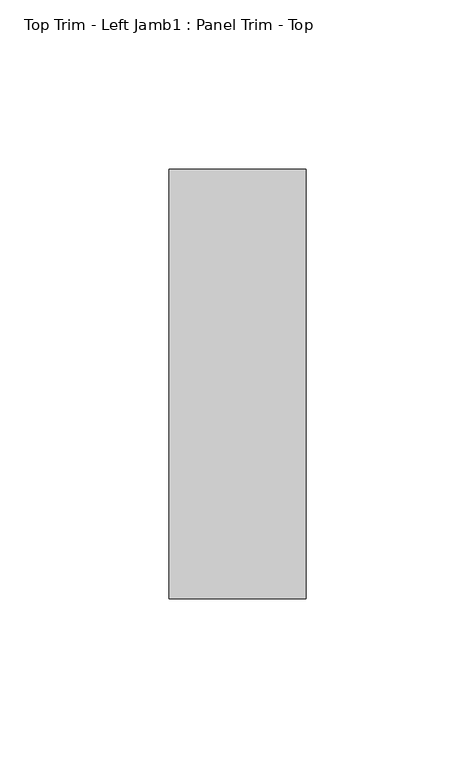
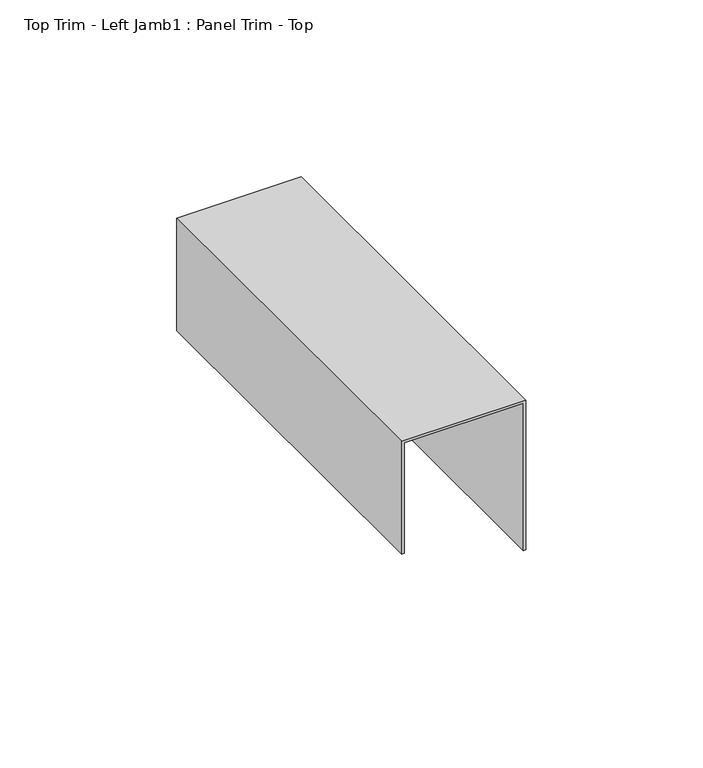
"""IFC4 building model written with IfcOpenShell, lengths in millimetres: proxy geometry, Top Trim - Left Jamb1 : Panel Trim - Top."""

import ifcopenshell
import ifcopenshell.guid

model = None  # the IFC model being written
_history = None  # IfcOwnerHistory: only IFC2X3 demands one
_inside = {}  # id of a spatial element -> (the spatial element, [elements in it])
_under = {}  # id of a project, library or spatial element -> (it, [spatial elements below it])
_declared = {}  # id of a project -> (the project, [libraries it declares])
_typed = {}  # id of a type object -> (the type object, [elements of that type])
_made_of = {}  # id of a material, layer set ... -> (it, [elements and type objects made of it])


def new_model(schema):
    """Start an empty IFC model of exactly this schema.

    Asked for "IFC4X3", IfcOpenShell would pick the latest addendum, in which some entities
    have other attributes; the version numbers below select the first issue.
    IFC2X3 requires an IfcOwnerHistory on every rooted entity: one is made here for all.
    """
    global model, _history
    if schema == "IFC4X3":
        model = ifcopenshell.file(schema_version=(4, 3, 0, 0))
    else:
        model = ifcopenshell.file(schema=schema)
    _inside.clear()
    _under.clear()
    _declared.clear()
    _typed.clear()
    _made_of.clear()
    _history = None
    if model.schema == "IFC2X3":
        org = make("IfcOrganization", Name="unknown")
        user = make(
            "IfcPersonAndOrganization",
            ThePerson=make("IfcPerson", FamilyName="unknown"),
            TheOrganization=org,
        )
        app = make(
            "IfcApplication",
            ApplicationDeveloper=org,
            Version="unknown",
            ApplicationFullName="unknown",
            ApplicationIdentifier="unknown",
        )
        _history = make(
            "IfcOwnerHistory",
            OwningUser=user,
            OwningApplication=app,
            ChangeAction="ADDED",
            CreationDate=0,
        )
    return model


def make(cls, **values):
    """One entity of the class cls with the attributes given. An attribute that is None is left unset."""
    return model.create_entity(
        cls, **{name: value for name, value in values.items() if value is not None}
    )


def rooted(cls, **values):
    """An entity with a GlobalId (a new one), such as an element, a storey or a relation."""
    return make(cls, GlobalId=ifcopenshell.guid.new(), OwnerHistory=_history, **values)


def si_unit(unit_type, name, prefix=None):
    """IfcSIUnit, for example si_unit("LENGTHUNIT", "METRE", prefix="MILLI")."""
    return make("IfcSIUnit", UnitType=unit_type, Prefix=prefix, Name=name)


def assignment(units):
    """IfcUnitAssignment: the units of a project."""
    return None if units is None else make("IfcUnitAssignment", Units=units)


def point(xyz):
    """IfcCartesianPoint."""
    return None if xyz is None else make("IfcCartesianPoint", Coordinates=xyz)


def direction(xyz):
    """IfcDirection."""
    return None if xyz is None else make("IfcDirection", DirectionRatios=xyz)


def frame(location, z_axis=None, x_axis=None):
    """IfcAxis2Placement3D, a coordinate frame: its origin and axes. An axis left out is left unset."""
    return make(
        "IfcAxis2Placement3D",
        Location=point(location),
        Axis=direction(z_axis),
        RefDirection=direction(x_axis),
    )


def origin():
    """The frame at (0, 0, 0) with its axes left unset."""
    return frame((0.0, 0.0, 0.0))


def place(relative_to, where):
    """IfcLocalPlacement: puts the frame where relative to a parent placement (None: the world)."""
    return make(
        "IfcLocalPlacement", PlacementRelTo=relative_to, RelativePlacement=where
    )


def context(
    kind, dimensions, precision=None, world=None, true_north=None, identifier=None
):
    """IfcGeometricRepresentationContext, for example the 3D "Model" context."""
    return make(
        "IfcGeometricRepresentationContext",
        ContextIdentifier=identifier,
        ContextType=kind,
        CoordinateSpaceDimension=dimensions,
        Precision=precision,
        WorldCoordinateSystem=world,
        TrueNorth=true_north,
    )


def project(units=None, contexts=None):
    """IfcProject with its units and contexts."""
    return rooted(
        "IfcProject",
        Name="project",
        RepresentationContexts=contexts,
        UnitsInContext=assignment(units),
    )


def spatial(cls, under=None, at=None, **own):
    """A site, building, storey or space (cls), placed at a placement, below another one or the project."""
    s = rooted(cls, ObjectPlacement=at, **own)
    if under is not None:
        _under.setdefault(under.id(), (under, []))[1].append(s)
    return s


def polyline(points):
    """IfcPolyline through the points."""
    return make("IfcPolyline", Points=[point(p) for p in points])


def outline(outer, holes=None, kind="AREA"):
    """IfcArbitraryClosedProfileDef: a profile drawn as a closed curve; with holes, ...WithVoids."""
    if holes is None:
        return make("IfcArbitraryClosedProfileDef", ProfileType=kind, OuterCurve=outer)
    return make(
        "IfcArbitraryProfileDefWithVoids",
        ProfileType=kind,
        OuterCurve=outer,
        InnerCurves=holes,
    )


def extrude(swept, where, along, depth):
    """IfcExtrudedAreaSolid: the profile swept, set in the frame where, extruded along a direction by depth."""
    return make(
        "IfcExtrudedAreaSolid",
        SweptArea=swept,
        Position=where,
        ExtrudedDirection=direction(along),
        Depth=depth,
    )


def shape(context_of_items, identifier, shape_type, items):
    """IfcShapeRepresentation: the items that make up one representation, for example the "Body"."""
    return make(
        "IfcShapeRepresentation",
        ContextOfItems=context_of_items,
        RepresentationIdentifier=identifier,
        RepresentationType=shape_type,
        Items=items,
    )


def source(mapping_origin, context_of_items, identifier, shape_type, items):
    """IfcRepresentationMap: a shape defined once, which mapped items show again and again."""
    return make(
        "IfcRepresentationMap",
        MappingOrigin=mapping_origin,
        MappedRepresentation=shape(context_of_items, identifier, shape_type, items),
    )


def transform(
    local_origin,
    x_axis=None,
    y_axis=None,
    z_axis=None,
    scale=None,
    scale2=None,
    scale3=None,
    uniform=True,
):
    """IfcCartesianTransformationOperator3D, or its non-uniform kind. x_axis, y_axis, z_axis: its Axis1, 2, 3."""
    if uniform:
        return make(
            "IfcCartesianTransformationOperator3D",
            Axis1=direction(x_axis),
            Axis2=direction(y_axis),
            LocalOrigin=point(local_origin),
            Scale=scale,
            Axis3=direction(z_axis),
        )
    return make(
        "IfcCartesianTransformationOperator3DnonUniform",
        Axis1=direction(x_axis),
        Axis2=direction(y_axis),
        LocalOrigin=point(local_origin),
        Scale=scale,
        Axis3=direction(z_axis),
        Scale2=scale2,
        Scale3=scale3,
    )


def mapped(mapping_source, mapping_target):
    """IfcMappedItem: shows the shape of a source again, moved by a transform."""
    return make(
        "IfcMappedItem", MappingSource=mapping_source, MappingTarget=mapping_target
    )


def made_of(thing, what):
    """Note that an element or type object is made of a material, layer set ...; save() writes the relation."""
    if what is not None:
        _made_of.setdefault(what.id(), (what, []))[1].append(thing)
    return thing


def element(
    cls,
    number,
    at=None,
    inside=None,
    cuts=None,
    type_object=None,
    material=None,
    context=None,
    identifier="Body",
    shape_type=None,
    held_by="IfcProductDefinitionShape",
    body=None,
    shapes=None,
    **own,
):
    """One element of the class cls, such as IfcWall. Its Tag is "e" and its number.

    at: its placement. inside: the storey or other place that contains it. cuts: it is an
    opening in that element (IfcRelVoidsElement). A single representation is given by context,
    identifier, shape_type and body (its items); several are given by shapes. held_by: the class
    of the entity that holds the representations. save() writes the other relations.
    """
    e = rooted(cls, Tag="e%d" % number, ObjectPlacement=at, **own)
    if body is not None:
        shapes = [shape(context, identifier, shape_type, body)]
    if shapes is not None:
        e.Representation = make(held_by, Representations=shapes)
    if inside is not None:
        _inside.setdefault(inside.id(), (inside, []))[1].append(e)
    if cuts is not None:
        rooted(
            "IfcRelVoidsElement", RelatingBuildingElement=cuts, RelatedOpeningElement=e
        )
    if type_object is not None:
        _typed.setdefault(type_object.id(), (type_object, []))[1].append(e)
    return made_of(e, material)


def aggregate(whole, parts):
    """IfcRelAggregates: a whole, such as a stair, and the parts it consists of."""
    return rooted("IfcRelAggregates", RelatingObject=whole, RelatedObjects=parts)


def save(model, path):
    """Write the relations noted so far, then the file.

    IfcRelAggregates (storeys below a building ...), IfcRelContainedInSpatialStructure (elements
    in a storey), IfcRelDefinesByType, IfcRelAssociatesMaterial and IfcRelDeclares: one each for
    every whole, place, type object, material and project.
    """
    for whole, parts in _under.values():
        aggregate(whole, parts)
    for where, things in _inside.values():
        rooted(
            "IfcRelContainedInSpatialStructure",
            RelatedElements=things,
            RelatingStructure=where,
        )
    for kind, things in _typed.values():
        rooted("IfcRelDefinesByType", RelatedObjects=things, RelatingType=kind)
    for what, things in _made_of.values():
        rooted("IfcRelAssociatesMaterial", RelatedObjects=things, RelatingMaterial=what)
    for by, libraries in _declared.values():
        rooted("IfcRelDeclares", RelatingContext=by, RelatedDefinitions=libraries)
    model.write(path)


def top_trim_left_jamb1_panel_trim_top_a1816676(model_context):
    return source(origin(), model_context, "Body", "SweptSolid", [
        extrude(outline(polyline([(2438.4, 587327.0060739), (2438.4, 587365.8934739), (2387.6, 587365.8934739), (2387.6, 587366.6808739), (2439.19375, 587366.6808739), (2439.19375, 587326.2186739), (2400.3, 587326.2186739), (2400.3, 587327.0060739), (2438.4, 587327.0060739)])), frame((0.0, -536420.7663841, 0.0), z_axis=(0.0, 1.0, 0.0), x_axis=(0.0, 0.0, 1.0)), (0.0, 0.0, 1.0), 127.0),
    ])


if __name__ == "__main__":
    model = new_model("IFC4")
    model_context = context("Model", 3, world=origin())
    ifc_project = project(units=[si_unit("LENGTHUNIT", "METRE", prefix="MILLI")], contexts=[model_context])
    site = spatial("IfcSite", under=ifc_project)
    building = spatial("IfcBuilding", under=site)
    placement = place(None, origin())
    top_trim_left_jamb1_panel_trim_top_shape = top_trim_left_jamb1_panel_trim_top_a1816676(model_context)
    element("IfcBuildingElementProxy", 1, Name="Top Trim - Left Jamb1 : Panel Trim - Top", ObjectType="Top Trim - Left Jamb1 : Panel Trim - Top", at=placement, inside=building, context=model_context, shape_type="MappedRepresentation", body=[
        mapped(top_trim_left_jamb1_panel_trim_top_shape, transform((0.0, 0.0, 0.0), x_axis=(1.0, 0.0, 0.0), y_axis=(0.0, 1.0, 0.0), z_axis=(0.0, 0.0, 1.0))),
    ])
    save(model, "model.ifc")

# Revit data of these elements
# Element 1 (IfcBuildingElementProxy, "Top Trim - Left Jamb1 : Panel Trim - Top")
#   Materials on its faces: "EDGE TRIM BY MTL PANEL MFR."
# Materials
#   "EDGE TRIM BY MTL PANEL MFR.": class "Generic", colour RGB 239 242 240, transparency 0, Cost = 0
